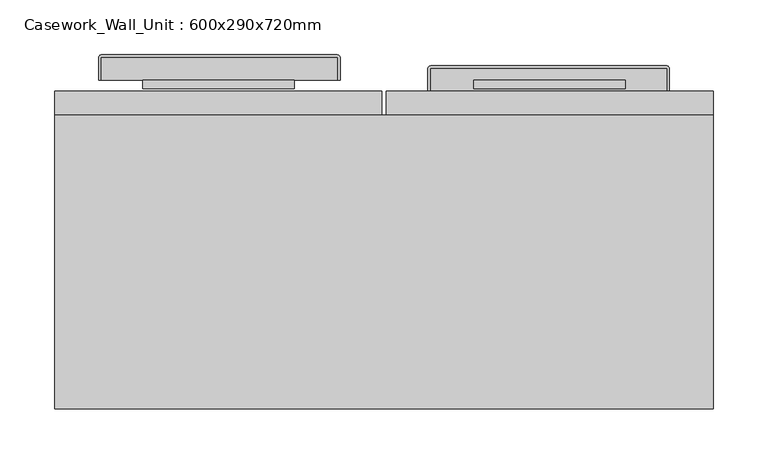
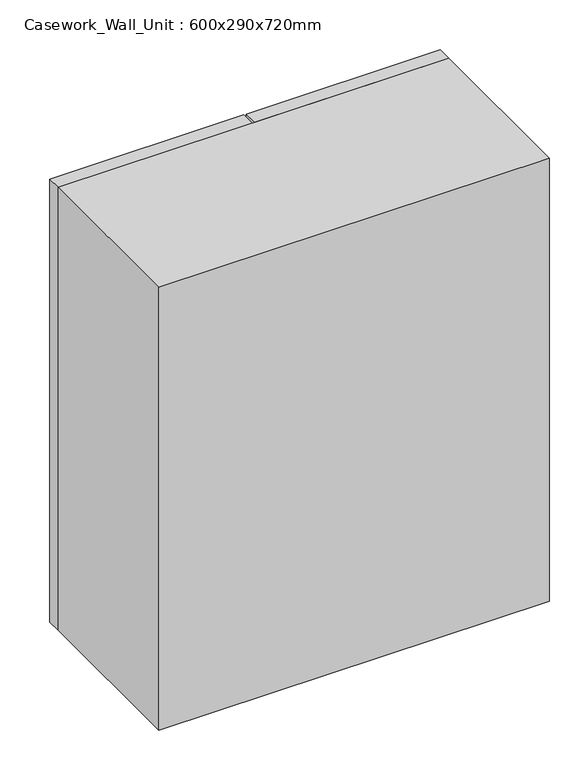
"""IFC4 building model written with IfcOpenShell, lengths in millimetres: furniture geometry, Casework_Wall_Unit : 600x290x720mm."""

from ifc_helpers import new_model, si_unit, point, frame, frame_2d, origin, place, context, project, spatial, polyline, circle_curve, trimmed, segment, composite_curve, outline, extrude, faceted_brep, source, transform, mapped, element, save


def casework_wall_unit_600x290x720mm_606a9a74(model_context):
    return source(origin(), model_context, "Body", "SolidModel", [
        extrude(outline(composite_curve([segment(polyline([(-83.0, 365.0), (-83.0, 385.5)]), True, "CONTINUOUS"), segment(trimmed(circle_curve(frame_2d((-82.5, 385.5)), 0.5), [point((-83.0, 385.5))], [point((-82.5, 386.0))], False, "CARTESIAN"), True, "CONTINUOUS"), segment(polyline([(-82.5, 386.0), (132.5, 386.0)]), True, "CONTINUOUS"), segment(trimmed(circle_curve(frame_2d((132.5, 385.5)), 0.5), [point((132.5, 386.0))], [point((133.0, 385.5))], False, "CARTESIAN"), True, "CONTINUOUS"), segment(polyline([(133.0, 385.5), (133.0, 365.0), (-83.0, 365.0)]), True, "CONTINUOUS")], self_intersect=False)), frame((0.0, 0.0, 1369.5509264), z_axis=(0.0, 0.0, 1.0), x_axis=(1.0, 0.0, 0.0)), (0.0, 0.0, 1.0), 6.4890959),
        extrude(outline(composite_curve([segment(polyline([(-85.0, 365.0), (-85.0, 385.5)]), True, "CONTINUOUS"), segment(trimmed(circle_curve(frame_2d((-82.5, 385.5)), 2.5), [point((-85.0, 385.5))], [point((-82.5, 388.0))], False, "CARTESIAN"), True, "CONTINUOUS"), segment(polyline([(-82.5, 388.0), (132.5, 388.0)]), True, "CONTINUOUS"), segment(trimmed(circle_curve(frame_2d((132.5, 385.5)), 2.5), [point((132.5, 388.0))], [point((135.0, 385.5))], False, "CARTESIAN"), True, "CONTINUOUS"), segment(polyline([(135.0, 385.5), (135.0, 365.0), (133.0, 365.0), (133.0, 385.5)]), True, "CONTINUOUS"), segment(trimmed(circle_curve(frame_2d((132.5, 385.5)), 0.5), [point((133.0, 385.5))], [point((132.5, 386.0))], True, "CARTESIAN"), True, "CONTINUOUS"), segment(polyline([(132.5, 386.0), (-82.5, 386.0)]), True, "CONTINUOUS"), segment(trimmed(circle_curve(frame_2d((-82.5, 385.5)), 0.5), [point((-82.5, 386.0))], [point((-83.0, 385.5))], True, "CARTESIAN"), True, "CONTINUOUS"), segment(polyline([(-83.0, 385.5), (-83.0, 365.0), (-85.0, 365.0)]), True, "CONTINUOUS")], self_intersect=False)), frame((0.0, 0.0, 1366.7855373), z_axis=(0.0, 0.0, 1.0), x_axis=(1.0, 0.0, 0.0)), (0.0, 0.0, 1.0), 12.0),
        extrude(outline(composite_curve([segment(polyline([(217.0, 355.0), (217.0, 375.5)]), True, "CONTINUOUS"), segment(trimmed(circle_curve(frame_2d((217.5, 375.5)), 0.5), [point((217.0, 375.5))], [point((217.5, 376.0))], False, "CARTESIAN"), True, "CONTINUOUS"), segment(polyline([(217.5, 376.0), (432.5, 376.0)]), True, "CONTINUOUS"), segment(trimmed(circle_curve(frame_2d((432.5, 375.5)), 0.5), [point((432.5, 376.0))], [point((433.0, 375.5))], False, "CARTESIAN"), True, "CONTINUOUS"), segment(polyline([(433.0, 375.5), (433.0, 355.0), (217.0, 355.0)]), True, "CONTINUOUS")], self_intersect=False)), frame((0.0, 0.0, 1369.5509264), z_axis=(0.0, 0.0, 1.0), x_axis=(1.0, 0.0, 0.0)), (0.0, 0.0, 1.0), 6.4890959),
        extrude(outline(composite_curve([segment(polyline([(215.0, 355.0), (215.0, 375.5)]), True, "CONTINUOUS"), segment(trimmed(circle_curve(frame_2d((217.5, 375.5)), 2.5), [point((215.0, 375.5))], [point((217.5, 378.0))], False, "CARTESIAN"), True, "CONTINUOUS"), segment(polyline([(217.5, 378.0), (432.5, 378.0)]), True, "CONTINUOUS"), segment(trimmed(circle_curve(frame_2d((432.5, 375.5)), 2.5), [point((432.5, 378.0))], [point((435.0, 375.5))], False, "CARTESIAN"), True, "CONTINUOUS"), segment(polyline([(435.0, 375.5), (435.0, 355.0), (433.0, 355.0), (433.0, 375.5)]), True, "CONTINUOUS"), segment(trimmed(circle_curve(frame_2d((432.5, 375.5)), 0.5), [point((433.0, 375.5))], [point((432.5, 376.0))], True, "CARTESIAN"), True, "CONTINUOUS"), segment(polyline([(432.5, 376.0), (217.5, 376.0)]), True, "CONTINUOUS"), segment(trimmed(circle_curve(frame_2d((217.5, 375.5)), 0.5), [point((217.5, 376.0))], [point((217.0, 375.5))], True, "CARTESIAN"), True, "CONTINUOUS"), segment(polyline([(217.0, 375.5), (217.0, 355.0), (215.0, 355.0)]), True, "CONTINUOUS")], self_intersect=False)), frame((0.0, 0.0, 1366.7855373), z_axis=(0.0, 0.0, 1.0), x_axis=(1.0, 0.0, 0.0)), (0.0, 0.0, 1.0), 12.0),
        extrude(outline(polyline([(395.0, 357.0), (257.0, 357.0), (257.0, 365.0), (395.0, 365.0), (395.0, 357.0)])), frame((0.0, 0.0, 1419.7855373), z_axis=(0.0, 0.0, 1.0), x_axis=(1.0, 0.0, 0.0)), (0.0, 0.0, 1.0), 540.0),
        extrude(outline(polyline([(93.0, 357.0), (-45.0, 357.0), (-45.0, 365.0), (93.0, 365.0), (93.0, 357.0)])), frame((0.0, 0.0, 1419.7855373), z_axis=(0.0, 0.0, 1.0), x_axis=(1.0, 0.0, 0.0)), (0.0, 0.0, 1.0), 540.0),
        faceted_brep([(453.0, 333.0, 1341.7855373), (-103.0, 333.0, 1341.7855373), (-103.0, 87.0, 1341.7855373), (453.0, 87.0, 1341.7855373), (475.0, 333.0, 1319.7855373), (475.0, 65.0, 1319.7855373), (-125.0, 65.0, 1319.7855373), (-125.0, 333.0, 1319.7855373), (-125.0, 333.0, 2039.7855373), (475.0, 333.0, 2039.7855373), (453.0, 333.0, 2017.7855373), (-103.0, 333.0, 2017.7855373), (-125.0, 65.0, 2039.7855373), (475.0, 65.0, 2039.7855373), (453.0, 87.0, 2017.7855373), (-103.0, 87.0, 2017.7855373)], [[[0, 1, 2, 3]], [[4, 5, 6, 7]], [[8, 9, 4, 7], [0, 10, 11, 1]], [[8, 7, 6, 12]], [[12, 6, 5, 13]], [[13, 5, 4, 9]], [[10, 0, 3, 14]], [[14, 3, 2, 15]], [[1, 11, 15, 2]], [[9, 8, 12, 13]], [[11, 10, 14, 15]]]),
        extrude(outline(polyline([(2039.7855373, 177.0), (1319.7855373, 177.0), (1319.7855373, 475.0), (2039.7855373, 475.0), (2039.7855373, 177.0)]), holes=[polyline([(1959.7855373, 257.0), (1959.7855373, 395.0), (1419.7855373, 395.0), (1419.7855373, 257.0), (1959.7855373, 257.0)])]), frame((0.0, 333.0, 0.0), z_axis=(0.0, 1.0, 0.0), x_axis=(0.0, 0.0, 1.0)), (0.0, 0.0, 1.0), 22.0),
        extrude(outline(polyline([(2039.7855373, 173.0), (2039.7855373, -125.0), (1319.7855373, -125.0), (1319.7855373, 173.0), (2039.7855373, 173.0)]), holes=[polyline([(1959.7855373, 93.0), (1419.7855373, 93.0), (1419.7855373, -45.0), (1959.7855373, -45.0), (1959.7855373, 93.0)])]), frame((0.0, 333.0, 0.0), z_axis=(0.0, 1.0, 0.0), x_axis=(0.0, 0.0, 1.0)), (0.0, 0.0, 1.0), 22.0),
    ])


if __name__ == "__main__":
    model = new_model("IFC4")
    model_context = context("Model", 3, world=origin())
    ifc_project = project(units=[si_unit("LENGTHUNIT", "METRE", prefix="MILLI")], contexts=[model_context])
    site = spatial("IfcSite", under=ifc_project)
    building = spatial("IfcBuilding", under=site)
    placement = place(None, origin())
    casework_wall_unit_600x290x720mm_shape = casework_wall_unit_600x290x720mm_606a9a74(model_context)
    element("IfcFurniture", 1, ObjectType="Casework_Wall_Unit : 600x290x720mm", at=placement, inside=building, context=model_context, shape_type="MappedRepresentation", body=[
        mapped(casework_wall_unit_600x290x720mm_shape, transform((0.0, 0.0, 0.0), x_axis=(1.0, 0.0, 0.0), y_axis=(0.0, 1.0, 0.0), z_axis=(0.0, 0.0, 1.0))),
    ])
    save(model, "model.ifc")

# Revit data of these elements
# Type "Casework_Wall_Unit : 600x290x720mm"
#   Manufacturer = "Revit"
#   Keynote = "N10"
#   Assembly Code = "C1030400"
#   Width = 600 mm
#   Height = 720 mm
#   Depth = 290 mm
#   Material Panel = Cabinets - Panel/Glass
#   Material Handle = Cabinets - Handles
#   Material Cabinet = Cabinets
# Element 1 (IfcFurniture, "Casework_Wall_Unit : 600x290x720mm")
#   Materials on its faces: "Cabinets - Handles", "Cabinets", "Cabinets - Panel/Glass"
# Materials
#   "Cabinets - Panel/Glass": class "Miscellaneous", colour RGB 252 255 255, transparency 0.72
#   "Cabinets - Handles": class "Metal", colour RGB 57 57 57, transparency 0
#   "Cabinets": class "Miscellaneous", colour RGB 249 249 249, transparency 0
